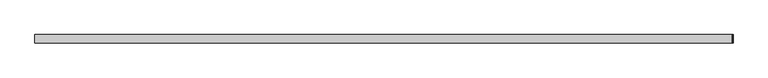
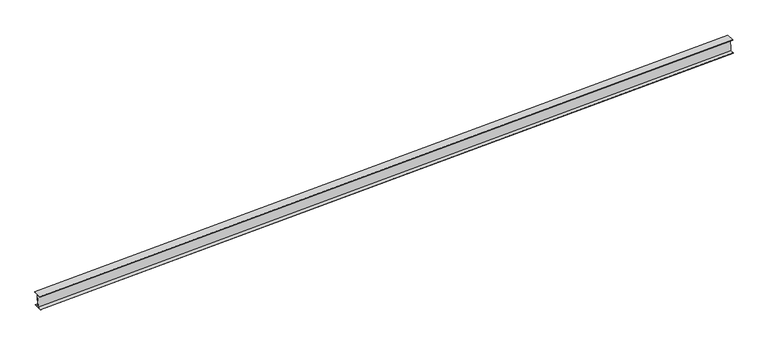
"""IFC4 building model written with IfcOpenShell, lengths in millimetres: proxy geometry, Generic Models 2:Generic Models 2:310765:Generic Models 2:310765 : Generic Models 2:Generic Models 2:310765:18 : Generic Models 2:Generic Models 2:310765:Generic Models 2:310765 : Generic Models 2:Generic Models 2:310765:300385."""

from ifc_helpers import new_model, si_unit, frame, origin, place, context, project, spatial, polyline, outline, extrude, source, transform, mapped, element, save


def generic_models_9332a2de(model_context):
    return source(origin(), model_context, "Body", "SweptSolid", [
        extrude(outline(polyline([(0.0, 0.0), (0.0, -6.858), (-152.4, -6.858), (-152.4, 0.0), (-79.121, 0.0), (-79.121, 240.2840001), (-152.4, 240.2840001), (-152.4, 247.142), (0.0, 247.142), (0.0, 240.2840001), (-73.025, 240.2840001), (-73.025, 0.0), (0.0, 0.0)])), frame((563169.680988, -578707.8428314, 3780.2261074), z_axis=(0.9991330730923568, 0.0, 0.04163054471206784), x_axis=(0.0, -1.0, 0.0)), (0.0, 0.0, 1.0), 12411.242059),
    ])


if __name__ == "__main__":
    model = new_model("IFC4")
    model_context = context("Model", 3, world=origin())
    ifc_project = project(units=[si_unit("LENGTHUNIT", "METRE", prefix="MILLI")], contexts=[model_context])
    site = spatial("IfcSite", under=ifc_project)
    building = spatial("IfcBuilding", under=site)
    placement = place(None, origin())
    generic_models_shape = generic_models_9332a2de(model_context)
    element("IfcBuildingElementProxy", 1, Name="Generic Models 2:Generic Models 2:310765:Generic Models 2:310765 : Generic Models 2:Generic Models 2:310765:18 : Generic Models 2:Generic Models 2:310765:Generic Models 2:310765 : Generic Models 2:Generic Models 2:310765:300385", ObjectType="Generic Models 2:Generic Models 2:310765:Generic Models 2:310765 : Generic Models 2:Generic Models 2:310765:18 : Generic Models 2:Generic Models 2:310765:Generic Models 2:310765 : Generic Models 2:Generic Models 2:310765:300385", at=placement, inside=building, context=model_context, shape_type="MappedRepresentation", body=[
        mapped(generic_models_shape, transform((0.0, 0.0, 0.0), x_axis=(1.0, 0.0, 0.0), y_axis=(0.0, 1.0, 0.0), z_axis=(0.0, 0.0, 1.0))),
    ])
    save(model, "model.ifc")

# Revit data of these elements
# Type "Generic Models 2:Generic Models 2:310765:Generic Models 2:310765 : Generic Models 2:Generic Models 2:310765:18 : Generic Models 2:Generic Models 2:310765:Generic Models 2:310765 : Generic Models 2:Generic Models 2:310765:300385"
#   NameOverride = "Generic Models 2:Generic Models 2:310765:Generic Models 2:310765 : Generic Models 2:Generic Models 2:310765:300385"
#   ObjectTypeOverride = "Generic Models 2:310765 : Generic Models 2:Generic Models 2:310765"
#   Reference = "Generic Models 2"
#   Tag = "300385"
# Element 1 (IfcBuildingElementProxy, "Generic Models 2:Generic Models 2:310765:Generic Models 2:310765 : Generic Models 2:Generic Models 2:310765:18 : Generic Models 2:Generic Models 2:310765:Generic Models 2:310765 : Generic Models 2:Generic Models 2:310765:300385")
#   Materials on its faces: "STRUCTURAL STEEL - SEE STRUCT. DWGS"
# Materials
#   "STRUCTURAL STEEL - SEE STRUCT. DWGS": class "Metal", colour RGB 189 187 185, transparency 0, Description = "Structural steel 50ksi", Cost = 0
